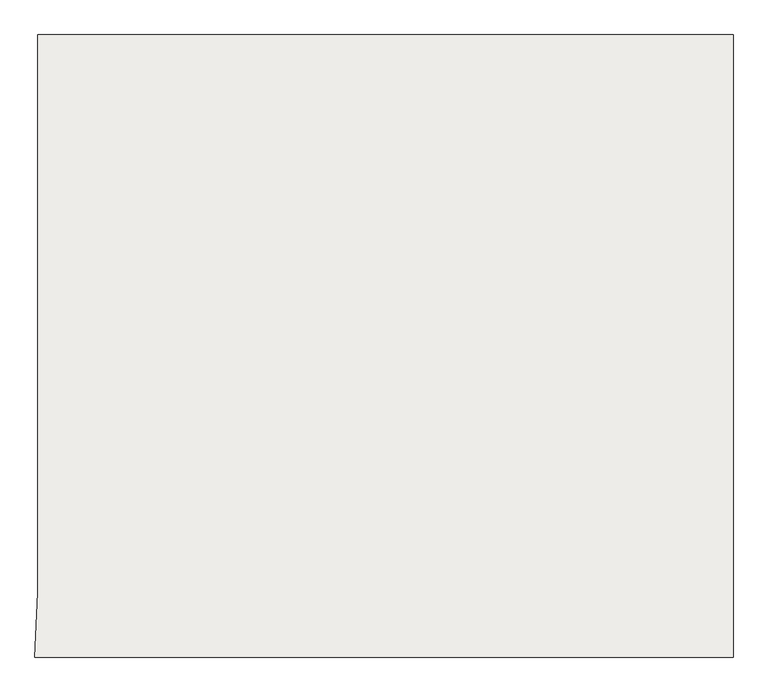
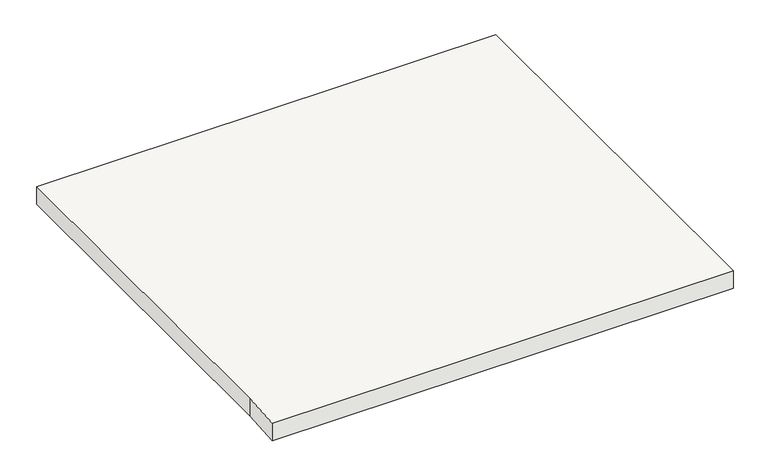
"""IFC4 building model written with IfcOpenShell, lengths in millimetres: slab geometry."""

from ifc_helpers import new_model, si_unit, frame, origin, place, context, project, spatial, polyline, outline, extrude, source, transform, mapped, element, save


def slab_18ee5c29(model_context):
    return source(origin(), model_context, "Body", "SweptSolid", [
        extrude(outline(polyline([(-11825.3533589, -8437.834784), (-10580.6631644, -8437.834784), (-10580.6631644, -9552.6519052), (-11830.6631644, -9552.6519052), (-11825.3533589, -9437.834784), (-11825.3533589, -8437.834784)])), frame((0.0, 0.0, 1443.3333333), z_axis=(0.0, 0.0, 1.0), x_axis=(1.0, 0.0, 0.0)), (0.0, 0.0, 1.0), 50.0),
    ])


if __name__ == "__main__":
    model = new_model("IFC4")
    model_context = context("Model", 3, world=origin())
    ifc_project = project(units=[si_unit("LENGTHUNIT", "METRE", prefix="MILLI")], contexts=[model_context])
    site = spatial("IfcSite", under=ifc_project)
    building = spatial("IfcBuilding", under=site)
    placement = place(None, origin())
    slab_shape = slab_18ee5c29(model_context)
    element("IfcSlab", 1, at=placement, inside=building, context=model_context, shape_type="MappedRepresentation", body=[
        mapped(slab_shape, transform((0.0, 0.0, 0.0), x_axis=(1.0, 0.0, 0.0), y_axis=(0.0, 1.0, 0.0), z_axis=(0.0, 0.0, 1.0))),
    ])
    save(model, "model.ifc")
